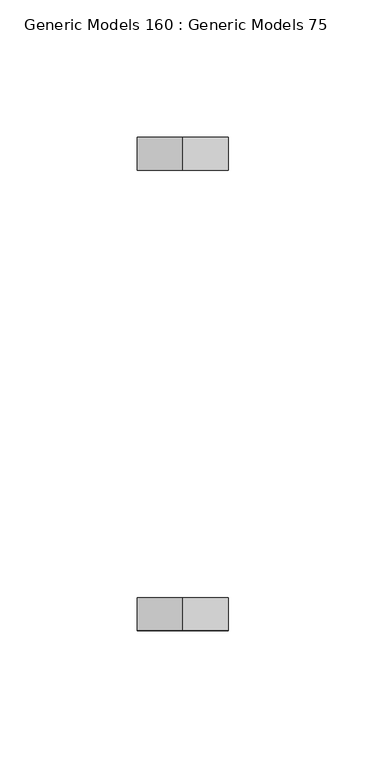
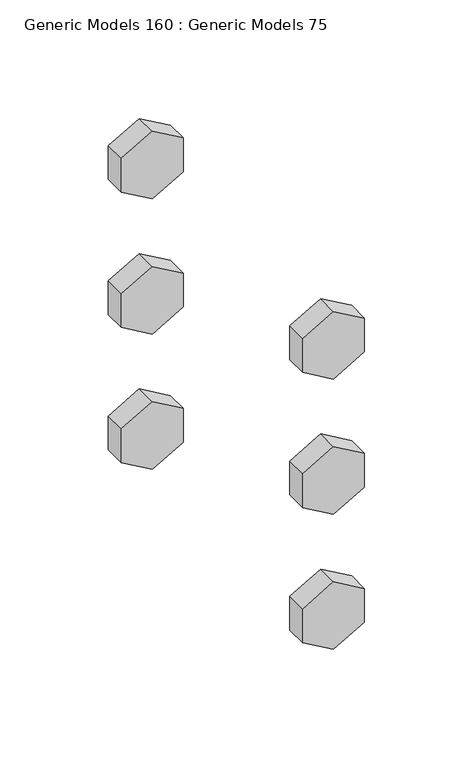
"""IFC4 building model written with IfcOpenShell, lengths in millimetres: proxy geometry, Generic Models 160 : Generic Models 75."""

from ifc_helpers import new_model, si_unit, frame, origin, place, context, project, spatial, polyline, outline, extrude, source, transform, mapped, element, save


def generic_models_160_generic_models_75_d1c9b105(model_context):
    return source(origin(), model_context, "Body", "SweptSolid", [
        extrude(outline(polyline([(271832.3875, 31689.0368192), (271822.8625, 31705.5346032), (271832.3875, 31722.0323871), (271851.4375, 31722.0323871), (271860.9625, 31705.5346032), (271851.4375, 31689.0368192), (271832.3875, 31689.0368192)])), frame((0.0, 36485.2082942, 0.0), z_axis=(0.0, 1.0, 0.0), x_axis=(0.0, 0.0, 1.0)), (0.0, 0.0, 1.0), 11.90625),
        extrude(outline(polyline([(271756.1875, 31689.0368192), (271746.6625, 31705.5346032), (271756.1875, 31722.0323871), (271775.2375, 31722.0323871), (271784.7625, 31705.5346032), (271775.2375, 31689.0368192), (271756.1875, 31689.0368192)])), frame((0.0, 36485.2082942, 0.0), z_axis=(0.0, 1.0, 0.0), x_axis=(0.0, 0.0, 1.0)), (0.0, 0.0, 1.0), 11.90625),
        extrude(outline(polyline([(271679.9875, 31689.0368192), (271670.4625, 31705.5346032), (271679.9875, 31722.0323871), (271699.0375, 31722.0323871), (271708.5625, 31705.5346032), (271699.0375, 31689.0368192), (271679.9875, 31689.0368192)])), frame((0.0, 36485.2082942, 0.0), z_axis=(0.0, 1.0, 0.0), x_axis=(0.0, 0.0, 1.0)), (0.0, 0.0, 1.0), 11.90625),
        extrude(outline(polyline([(271832.3875, 31689.0368192), (271822.8625, 31705.5346032), (271832.3875, 31722.0323871), (271851.4375, 31722.0323871), (271860.9625, 31705.5346032), (271851.4375, 31689.0368192), (271832.3875, 31689.0368192)])), frame((0.0, 36317.7270442, 0.0), z_axis=(0.0, 1.0, 0.0), x_axis=(0.0, 0.0, 1.0)), (0.0, 0.0, 1.0), 11.90625),
        extrude(outline(polyline([(271756.1875, 31689.0368192), (271746.6625, 31705.5346032), (271756.1875, 31722.0323871), (271775.2375, 31722.0323871), (271784.7625, 31705.5346032), (271775.2375, 31689.0368192), (271756.1875, 31689.0368192)])), frame((0.0, 36317.7270442, 0.0), z_axis=(0.0, 1.0, 0.0), x_axis=(0.0, 0.0, 1.0)), (0.0, 0.0, 1.0), 11.90625),
        extrude(outline(polyline([(271679.9875, 31689.0368192), (271670.4625, 31705.5346032), (271679.9875, 31722.0323871), (271699.0375, 31722.0323871), (271708.5625, 31705.5346032), (271699.0375, 31689.0368192), (271679.9875, 31689.0368192)])), frame((0.0, 36317.7270442, 0.0), z_axis=(0.0, 1.0, 0.0), x_axis=(0.0, 0.0, 1.0)), (0.0, 0.0, 1.0), 11.90625),
    ])


if __name__ == "__main__":
    model = new_model("IFC4")
    model_context = context("Model", 3, world=origin())
    ifc_project = project(units=[si_unit("LENGTHUNIT", "METRE", prefix="MILLI")], contexts=[model_context])
    site = spatial("IfcSite", under=ifc_project)
    building = spatial("IfcBuilding", under=site)
    placement = place(None, origin())
    generic_models_160_generic_models_75_shape = generic_models_160_generic_models_75_d1c9b105(model_context)
    element("IfcBuildingElementProxy", 1, Name="Generic Models 160 : Generic Models 75", ObjectType="Generic Models 160 : Generic Models 75", at=placement, inside=building, context=model_context, shape_type="MappedRepresentation", body=[
        mapped(generic_models_160_generic_models_75_shape, transform((0.0, 0.0, 0.0), x_axis=(1.0, 0.0, 0.0), y_axis=(0.0, 1.0, 0.0), z_axis=(0.0, 0.0, 1.0))),
    ])
    save(model, "model.ifc")
